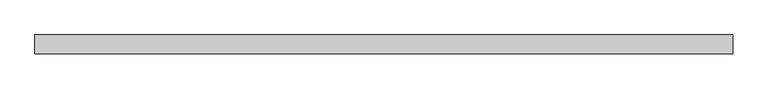
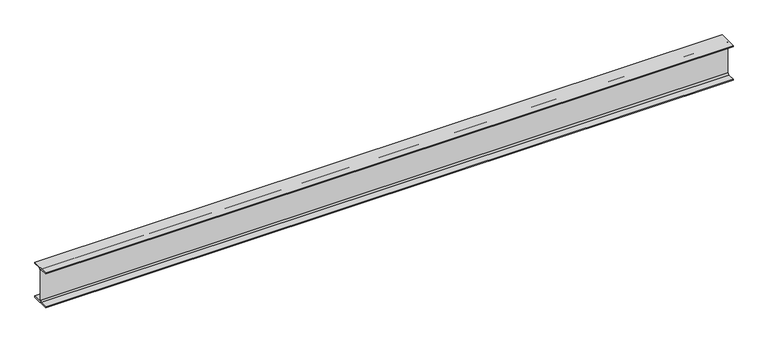
"""IFC4 building model written with IfcOpenShell, lengths in millimetres: beam geometry, Steel Framing_H_KS : H_SB_AR_S02_H-300x150x6.5x9_SRB3."""

import ifcopenshell
import ifcopenshell.guid

model = None  # the IFC model being written
_history = None  # IfcOwnerHistory: only IFC2X3 demands one
_inside = {}  # id of a spatial element -> (the spatial element, [elements in it])
_under = {}  # id of a project, library or spatial element -> (it, [spatial elements below it])
_declared = {}  # id of a project -> (the project, [libraries it declares])
_typed = {}  # id of a type object -> (the type object, [elements of that type])
_made_of = {}  # id of a material, layer set ... -> (it, [elements and type objects made of it])


def new_model(schema):
    """Start an empty IFC model of exactly this schema.

    Asked for "IFC4X3", IfcOpenShell would pick the latest addendum, in which some entities
    have other attributes; the version numbers below select the first issue.
    IFC2X3 requires an IfcOwnerHistory on every rooted entity: one is made here for all.
    """
    global model, _history
    if schema == "IFC4X3":
        model = ifcopenshell.file(schema_version=(4, 3, 0, 0))
    else:
        model = ifcopenshell.file(schema=schema)
    _inside.clear()
    _under.clear()
    _declared.clear()
    _typed.clear()
    _made_of.clear()
    _history = None
    if model.schema == "IFC2X3":
        org = make("IfcOrganization", Name="unknown")
        user = make(
            "IfcPersonAndOrganization",
            ThePerson=make("IfcPerson", FamilyName="unknown"),
            TheOrganization=org,
        )
        app = make(
            "IfcApplication",
            ApplicationDeveloper=org,
            Version="unknown",
            ApplicationFullName="unknown",
            ApplicationIdentifier="unknown",
        )
        _history = make(
            "IfcOwnerHistory",
            OwningUser=user,
            OwningApplication=app,
            ChangeAction="ADDED",
            CreationDate=0,
        )
    return model


def make(cls, **values):
    """One entity of the class cls with the attributes given. An attribute that is None is left unset."""
    return model.create_entity(
        cls, **{name: value for name, value in values.items() if value is not None}
    )


def rooted(cls, **values):
    """An entity with a GlobalId (a new one), such as an element, a storey or a relation."""
    return make(cls, GlobalId=ifcopenshell.guid.new(), OwnerHistory=_history, **values)


def si_unit(unit_type, name, prefix=None):
    """IfcSIUnit, for example si_unit("LENGTHUNIT", "METRE", prefix="MILLI")."""
    return make("IfcSIUnit", UnitType=unit_type, Prefix=prefix, Name=name)


def assignment(units):
    """IfcUnitAssignment: the units of a project."""
    return None if units is None else make("IfcUnitAssignment", Units=units)


def point(xyz):
    """IfcCartesianPoint."""
    return None if xyz is None else make("IfcCartesianPoint", Coordinates=xyz)


def direction(xyz):
    """IfcDirection."""
    return None if xyz is None else make("IfcDirection", DirectionRatios=xyz)


def frame(location, z_axis=None, x_axis=None):
    """IfcAxis2Placement3D, a coordinate frame: its origin and axes. An axis left out is left unset."""
    return make(
        "IfcAxis2Placement3D",
        Location=point(location),
        Axis=direction(z_axis),
        RefDirection=direction(x_axis),
    )


def frame_2d(location, x_axis=None):
    """IfcAxis2Placement2D, a coordinate frame in the plane: its origin and x axis."""
    return make(
        "IfcAxis2Placement2D", Location=point(location), RefDirection=direction(x_axis)
    )


def origin():
    """The frame at (0, 0, 0) with its axes left unset."""
    return frame((0.0, 0.0, 0.0))


def place(relative_to, where):
    """IfcLocalPlacement: puts the frame where relative to a parent placement (None: the world)."""
    return make(
        "IfcLocalPlacement", PlacementRelTo=relative_to, RelativePlacement=where
    )


def context(
    kind, dimensions, precision=None, world=None, true_north=None, identifier=None
):
    """IfcGeometricRepresentationContext, for example the 3D "Model" context."""
    return make(
        "IfcGeometricRepresentationContext",
        ContextIdentifier=identifier,
        ContextType=kind,
        CoordinateSpaceDimension=dimensions,
        Precision=precision,
        WorldCoordinateSystem=world,
        TrueNorth=true_north,
    )


def project(units=None, contexts=None):
    """IfcProject with its units and contexts."""
    return rooted(
        "IfcProject",
        Name="project",
        RepresentationContexts=contexts,
        UnitsInContext=assignment(units),
    )


def spatial(cls, under=None, at=None, **own):
    """A site, building, storey or space (cls), placed at a placement, below another one or the project."""
    s = rooted(cls, ObjectPlacement=at, **own)
    if under is not None:
        _under.setdefault(under.id(), (under, []))[1].append(s)
    return s


def polyline(points):
    """IfcPolyline through the points."""
    return make("IfcPolyline", Points=[point(p) for p in points])


def circle_curve(where, radius):
    """IfcCircle in the frame where."""
    return make("IfcCircle", Position=where, Radius=radius)


def trimmed(basis, trim1, trim2, sense, master):
    """IfcTrimmedCurve: the piece of a basis curve between two trims."""
    return make(
        "IfcTrimmedCurve",
        BasisCurve=basis,
        Trim1=trim1,
        Trim2=trim2,
        SenseAgreement=sense,
        MasterRepresentation=master,
    )


def segment(curve, same_sense, transition):
    """IfcCompositeCurveSegment."""
    return make(
        "IfcCompositeCurveSegment",
        Transition=transition,
        SameSense=same_sense,
        ParentCurve=curve,
    )


def composite_curve(segments, self_intersect=None):
    """IfcCompositeCurve: segments joined end to end."""
    return make("IfcCompositeCurve", Segments=segments, SelfIntersect=self_intersect)


def outline(outer, holes=None, kind="AREA"):
    """IfcArbitraryClosedProfileDef: a profile drawn as a closed curve; with holes, ...WithVoids."""
    if holes is None:
        return make("IfcArbitraryClosedProfileDef", ProfileType=kind, OuterCurve=outer)
    return make(
        "IfcArbitraryProfileDefWithVoids",
        ProfileType=kind,
        OuterCurve=outer,
        InnerCurves=holes,
    )


def extrude(swept, where, along, depth):
    """IfcExtrudedAreaSolid: the profile swept, set in the frame where, extruded along a direction by depth."""
    return make(
        "IfcExtrudedAreaSolid",
        SweptArea=swept,
        Position=where,
        ExtrudedDirection=direction(along),
        Depth=depth,
    )


def shape(context_of_items, identifier, shape_type, items):
    """IfcShapeRepresentation: the items that make up one representation, for example the "Body"."""
    return make(
        "IfcShapeRepresentation",
        ContextOfItems=context_of_items,
        RepresentationIdentifier=identifier,
        RepresentationType=shape_type,
        Items=items,
    )


def source(mapping_origin, context_of_items, identifier, shape_type, items):
    """IfcRepresentationMap: a shape defined once, which mapped items show again and again."""
    return make(
        "IfcRepresentationMap",
        MappingOrigin=mapping_origin,
        MappedRepresentation=shape(context_of_items, identifier, shape_type, items),
    )


def transform(
    local_origin,
    x_axis=None,
    y_axis=None,
    z_axis=None,
    scale=None,
    scale2=None,
    scale3=None,
    uniform=True,
):
    """IfcCartesianTransformationOperator3D, or its non-uniform kind. x_axis, y_axis, z_axis: its Axis1, 2, 3."""
    if uniform:
        return make(
            "IfcCartesianTransformationOperator3D",
            Axis1=direction(x_axis),
            Axis2=direction(y_axis),
            LocalOrigin=point(local_origin),
            Scale=scale,
            Axis3=direction(z_axis),
        )
    return make(
        "IfcCartesianTransformationOperator3DnonUniform",
        Axis1=direction(x_axis),
        Axis2=direction(y_axis),
        LocalOrigin=point(local_origin),
        Scale=scale,
        Axis3=direction(z_axis),
        Scale2=scale2,
        Scale3=scale3,
    )


def mapped(mapping_source, mapping_target):
    """IfcMappedItem: shows the shape of a source again, moved by a transform."""
    return make(
        "IfcMappedItem", MappingSource=mapping_source, MappingTarget=mapping_target
    )


def made_of(thing, what):
    """Note that an element or type object is made of a material, layer set ...; save() writes the relation."""
    if what is not None:
        _made_of.setdefault(what.id(), (what, []))[1].append(thing)
    return thing


def element(
    cls,
    number,
    at=None,
    inside=None,
    cuts=None,
    type_object=None,
    material=None,
    context=None,
    identifier="Body",
    shape_type=None,
    held_by="IfcProductDefinitionShape",
    body=None,
    shapes=None,
    **own,
):
    """One element of the class cls, such as IfcWall. Its Tag is "e" and its number.

    at: its placement. inside: the storey or other place that contains it. cuts: it is an
    opening in that element (IfcRelVoidsElement). A single representation is given by context,
    identifier, shape_type and body (its items); several are given by shapes. held_by: the class
    of the entity that holds the representations. save() writes the other relations.
    """
    e = rooted(cls, Tag="e%d" % number, ObjectPlacement=at, **own)
    if body is not None:
        shapes = [shape(context, identifier, shape_type, body)]
    if shapes is not None:
        e.Representation = make(held_by, Representations=shapes)
    if inside is not None:
        _inside.setdefault(inside.id(), (inside, []))[1].append(e)
    if cuts is not None:
        rooted(
            "IfcRelVoidsElement", RelatingBuildingElement=cuts, RelatedOpeningElement=e
        )
    if type_object is not None:
        _typed.setdefault(type_object.id(), (type_object, []))[1].append(e)
    return made_of(e, material)


def aggregate(whole, parts):
    """IfcRelAggregates: a whole, such as a stair, and the parts it consists of."""
    return rooted("IfcRelAggregates", RelatingObject=whole, RelatedObjects=parts)


def save(model, path):
    """Write the relations noted so far, then the file.

    IfcRelAggregates (storeys below a building ...), IfcRelContainedInSpatialStructure (elements
    in a storey), IfcRelDefinesByType, IfcRelAssociatesMaterial and IfcRelDeclares: one each for
    every whole, place, type object, material and project.
    """
    for whole, parts in _under.values():
        aggregate(whole, parts)
    for where, things in _inside.values():
        rooted(
            "IfcRelContainedInSpatialStructure",
            RelatedElements=things,
            RelatingStructure=where,
        )
    for kind, things in _typed.values():
        rooted("IfcRelDefinesByType", RelatedObjects=things, RelatingType=kind)
    for what, things in _made_of.values():
        rooted("IfcRelAssociatesMaterial", RelatedObjects=things, RelatingMaterial=what)
    for by, libraries in _declared.values():
        rooted("IfcRelDeclares", RelatingContext=by, RelatedDefinitions=libraries)
    model.write(path)


def beam_48b2d694(model_context):
    return source(origin(), model_context, "Body", "SweptSolid", [
        extrude(outline(composite_curve([segment(polyline([(75.0, -141.0), (75.0, -150.0), (-75.0, -150.0), (-75.0, -141.0), (-16.25, -141.0)]), True, "CONTINUOUS"), segment(trimmed(circle_curve(frame_2d((-16.25, -128.0)), 13.0), [point((-16.25, -141.0))], [point((-3.25, -128.0))], True, "CARTESIAN"), True, "CONTINUOUS"), segment(polyline([(-3.25, -128.0), (-3.25, 128.0)]), True, "CONTINUOUS"), segment(trimmed(circle_curve(frame_2d((-16.25, 128.0)), 13.0), [point((-3.25, 128.0))], [point((-16.25, 141.0))], True, "CARTESIAN"), True, "CONTINUOUS"), segment(polyline([(-16.25, 141.0), (-75.0, 141.0), (-75.0, 150.0), (75.0, 150.0), (75.0, 141.0), (16.25, 141.0)]), True, "CONTINUOUS"), segment(trimmed(circle_curve(frame_2d((16.25, 128.0)), 13.0), [point((16.25, 141.0))], [point((3.25, 128.0))], True, "CARTESIAN"), True, "CONTINUOUS"), segment(polyline([(3.25, 128.0), (3.25, -128.0)]), True, "CONTINUOUS"), segment(trimmed(circle_curve(frame_2d((16.25, -128.0)), 13.0), [point((3.25, -128.0))], [point((16.25, -141.0))], True, "CARTESIAN"), True, "CONTINUOUS"), segment(polyline([(16.25, -141.0), (75.0, -141.0)]), True, "CONTINUOUS")], self_intersect=False)), frame((-2693.3, 0.0, 0.0), z_axis=(1.0, 0.0, 0.0), x_axis=(0.0, 1.0, 0.0)), (0.0, 0.0, 1.0), 5580.6),
    ])


if __name__ == "__main__":
    model = new_model("IFC4")
    model_context = context("Model", 3, world=origin())
    ifc_project = project(units=[si_unit("LENGTHUNIT", "METRE", prefix="MILLI")], contexts=[model_context])
    site = spatial("IfcSite", under=ifc_project)
    building = spatial("IfcBuilding", under=site)
    placement = place(None, origin())
    beam_shape = beam_48b2d694(model_context)
    element("IfcBeam", 1, ObjectType="Steel Framing_H_KS : H_SB_AR_S02_H-300x150x6.5x9_SRB3", at=placement, inside=building, context=model_context, shape_type="MappedRepresentation", body=[
        mapped(beam_shape, transform((0.0, 0.0, 0.0), x_axis=(1.0, 0.0, 0.0), y_axis=(0.0, 1.0, 0.0), z_axis=(0.0, 0.0, 1.0))),
    ])
    save(model, "model.ifc")

# Revit data of these elements
# Type "Steel Framing_H_KS : H_SB_AR_S02_H-300x150x6.5x9_SRB3"
#   Type Comments = "MAIN"
#   Type Mark = "SRB3"
#   H_SectionID = "H-300x150x6.5x9"
#   H_Ratio for Additional Steel Plate = 0.2
#   Width = 15.0 cm
#   Web Thickness = 0.65 cm
#   Web Fillet = 1.3 cm
#   Warping Constant = 107000.0 cm⁶
#   Torsional Moment of Inertia = 9.9539 cm⁴
#   Section Area = 46.78 cm²
#   Plastic Modulus weak axis = 105.0 cm³
#   Plastic Modulus strong axis = 542.0 cm³
#   Perimeter = 1.17 m²/m
#   Nominal Weight = 36.70 kgf/m
#   Moment of Inertia weak axis = 508.00 cm⁴
#   Moment of Inertia strong axis = 7210.00 cm⁴
#   Height = 30.0 cm
#   Flange Thickness = 0.9 cm
#   Elastic Modulus weak axis = 67.7 cm³
#   Elastic Modulus strong axis = 481.0 cm³
#   Centroid Vertical = 15.0 cm
#   Centroid Horizontal = 7.5 cm
#   Bolt Spacing = 8.89 cm
#   Length [instance default] = 1500 mm
#   Structural Material [instance default] = Steel, 45-345
#   Section Name Key = ""
#   Assembly Code = ""
# Element 1 (IfcBeam, "Steel Framing_H_KS : H_SB_AR_S02_H-300x150x6.5x9_SRB3")
#   Materials on its faces: "Steel, 45-345"
# Materials
#   "Steel, 45-345": class "Metal", colour RGB 189 187 185, transparency 0, Description = "Steel 345 MPa", Cost = 0
